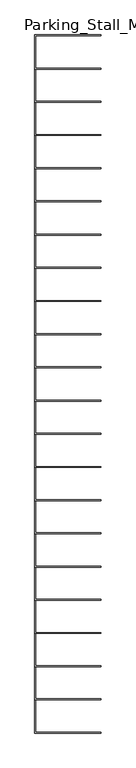
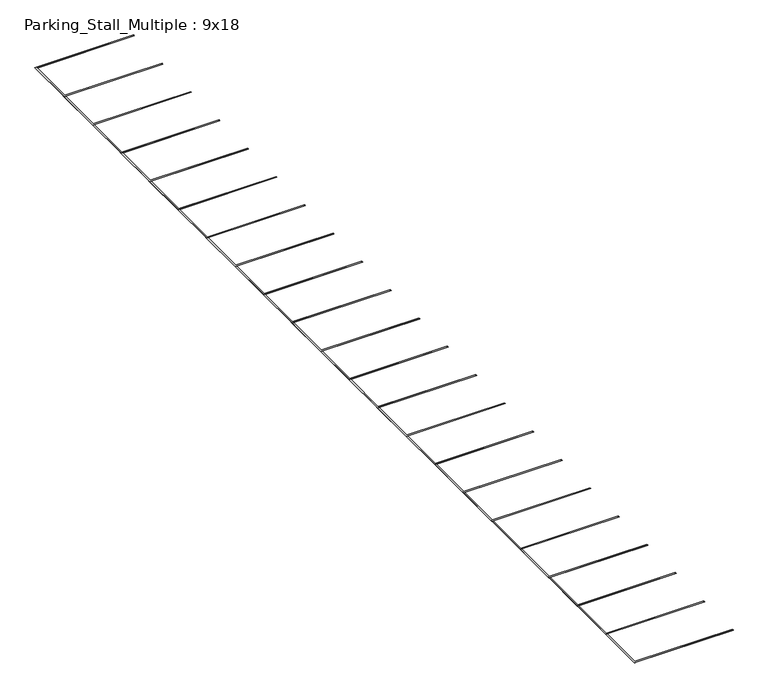
"""IFC4 building model written with IfcOpenShell, lengths in millimetres: proxy geometry, Parking_Stall_Multiple : 9x18."""

from ifc_helpers import new_model, si_unit, origin, origin_with_axes, place, context, project, spatial, polyline, outline, extrude, source, transform, mapped, element, save


def parking_stall_multiple_9x18_b0386777(model_context):
    return source(origin(), model_context, "Body", "SweptSolid", [
        extrude(outline(polyline([(5486.4, 54864.0), (0.0, 54864.0), (0.0, 57683.4), (5486.4, 57683.4), (5486.4, 57607.2), (76.2, 57607.2), (76.2, 54940.2), (5486.4, 54940.2), (5486.4, 54864.0)])), origin_with_axes(), (0.0, 0.0, 1.0), 6.35),
        extrude(outline(polyline([(5486.4, 52120.8), (0.0, 52120.8), (0.0, 54940.2), (5486.4, 54940.2), (5486.4, 54864.0), (76.2, 54864.0), (76.2, 52197.0), (5486.4, 52197.0), (5486.4, 52120.8)])), origin_with_axes(), (0.0, 0.0, 1.0), 6.35),
        extrude(outline(polyline([(5486.4, 49377.6), (0.0, 49377.6), (0.0, 52197.0), (5486.4, 52197.0), (5486.4, 52120.8), (76.2, 52120.8), (76.2, 49453.8), (5486.4, 49453.8), (5486.4, 49377.6)])), origin_with_axes(), (0.0, 0.0, 1.0), 6.35),
        extrude(outline(polyline([(5486.4, 46634.4), (0.0, 46634.4), (0.0, 49453.8), (5486.4, 49453.8), (5486.4, 49377.6), (76.2, 49377.6), (76.2, 46710.6), (5486.4, 46710.6), (5486.4, 46634.4)])), origin_with_axes(), (0.0, 0.0, 1.0), 6.35),
        extrude(outline(polyline([(5486.4, 43891.2), (0.0, 43891.2), (0.0, 46710.6), (5486.4, 46710.6), (5486.4, 46634.4), (76.2, 46634.4), (76.2, 43967.4), (5486.4, 43967.4), (5486.4, 43891.2)])), origin_with_axes(), (0.0, 0.0, 1.0), 6.35),
        extrude(outline(polyline([(5486.4, 41148.0), (0.0, 41148.0), (0.0, 43967.4), (5486.4, 43967.4), (5486.4, 43891.2), (76.2, 43891.2), (76.2, 41224.2), (5486.4, 41224.2), (5486.4, 41148.0)])), origin_with_axes(), (0.0, 0.0, 1.0), 6.35),
        extrude(outline(polyline([(5486.4, 38404.8), (0.0, 38404.8), (0.0, 41224.2), (5486.4, 41224.2), (5486.4, 41148.0), (76.2, 41148.0), (76.2, 38481.0), (5486.4, 38481.0), (5486.4, 38404.8)])), origin_with_axes(), (0.0, 0.0, 1.0), 6.35),
        extrude(outline(polyline([(5486.4, 35661.6), (0.0, 35661.6), (0.0, 38481.0), (5486.4, 38481.0), (5486.4, 38404.8), (76.2, 38404.8), (76.2, 35737.8), (5486.4, 35737.8), (5486.4, 35661.6)])), origin_with_axes(), (0.0, 0.0, 1.0), 6.35),
        extrude(outline(polyline([(5486.4, 32918.4), (0.0, 32918.4), (0.0, 35737.8), (5486.4, 35737.8), (5486.4, 35661.6), (76.2, 35661.6), (76.2, 32994.6), (5486.4, 32994.6), (5486.4, 32918.4)])), origin_with_axes(), (0.0, 0.0, 1.0), 6.35),
        extrude(outline(polyline([(5486.4, 30175.2), (0.0, 30175.2), (0.0, 32994.6), (5486.4, 32994.6), (5486.4, 32918.4), (76.2, 32918.4), (76.2, 30251.4), (5486.4, 30251.4), (5486.4, 30175.2)])), origin_with_axes(), (0.0, 0.0, 1.0), 6.35),
        extrude(outline(polyline([(5486.4, 27432.0), (0.0, 27432.0), (0.0, 30251.4), (5486.4, 30251.4), (5486.4, 30175.2), (76.2, 30175.2), (76.2, 27508.2), (5486.4, 27508.2), (5486.4, 27432.0)])), origin_with_axes(), (0.0, 0.0, 1.0), 6.35),
        extrude(outline(polyline([(5486.4, 24688.8), (0.0, 24688.8), (0.0, 27508.2), (5486.4, 27508.2), (5486.4, 27432.0), (76.2, 27432.0), (76.2, 24765.0), (5486.4, 24765.0), (5486.4, 24688.8)])), origin_with_axes(), (0.0, 0.0, 1.0), 6.35),
        extrude(outline(polyline([(5486.4, 21945.6), (0.0, 21945.6), (0.0, 24765.0), (5486.4, 24765.0), (5486.4, 24688.8), (76.2, 24688.8), (76.2, 22021.8), (5486.4, 22021.8), (5486.4, 21945.6)])), origin_with_axes(), (0.0, 0.0, 1.0), 6.35),
        extrude(outline(polyline([(5486.4, 19202.4), (0.0, 19202.4), (0.0, 22021.8), (5486.4, 22021.8), (5486.4, 21945.6), (76.2, 21945.6), (76.2, 19278.6), (5486.4, 19278.6), (5486.4, 19202.4)])), origin_with_axes(), (0.0, 0.0, 1.0), 6.35),
        extrude(outline(polyline([(5486.4, 16459.2), (0.0, 16459.2), (0.0, 19278.6), (5486.4, 19278.6), (5486.4, 19202.4), (76.2, 19202.4), (76.2, 16535.4), (5486.4, 16535.4), (5486.4, 16459.2)])), origin_with_axes(), (0.0, 0.0, 1.0), 6.35),
        extrude(outline(polyline([(5486.4, 13716.0), (0.0, 13716.0), (0.0, 16535.4), (5486.4, 16535.4), (5486.4, 16459.2), (76.2, 16459.2), (76.2, 13792.2), (5486.4, 13792.2), (5486.4, 13716.0)])), origin_with_axes(), (0.0, 0.0, 1.0), 6.35),
        extrude(outline(polyline([(5486.4, 10972.8), (0.0, 10972.8), (0.0, 13792.2), (5486.4, 13792.2), (5486.4, 13716.0), (76.2, 13716.0), (76.2, 11049.0), (5486.4, 11049.0), (5486.4, 10972.8)])), origin_with_axes(), (0.0, 0.0, 1.0), 6.35),
        extrude(outline(polyline([(5486.4, 8229.6), (0.0, 8229.6), (0.0, 11049.0), (5486.4, 11049.0), (5486.4, 10972.8), (76.2, 10972.8), (76.2, 8305.8), (5486.4, 8305.8), (5486.4, 8229.6)])), origin_with_axes(), (0.0, 0.0, 1.0), 6.35),
        extrude(outline(polyline([(5486.4, 5486.4), (0.0, 5486.4), (0.0, 8305.8), (5486.4, 8305.8), (5486.4, 8229.6), (76.2, 8229.6), (76.2, 5562.6), (5486.4, 5562.6), (5486.4, 5486.4)])), origin_with_axes(), (0.0, 0.0, 1.0), 6.35),
        extrude(outline(polyline([(5486.4, 2743.2), (0.0, 2743.2), (0.0, 5562.6), (5486.4, 5562.6), (5486.4, 5486.4), (76.2, 5486.4), (76.2, 2819.4), (5486.4, 2819.4), (5486.4, 2743.2)])), origin_with_axes(), (0.0, 0.0, 1.0), 6.35),
        extrude(outline(polyline([(5486.4, 0.0), (0.0, 0.0), (0.0, 2819.4), (5486.4, 2819.4), (5486.4, 2743.2), (76.2, 2743.2), (76.2, 76.2), (5486.4, 76.2), (5486.4, 0.0)])), origin_with_axes(), (0.0, 0.0, 1.0), 6.35),
    ])


if __name__ == "__main__":
    model = new_model("IFC4")
    model_context = context("Model", 3, world=origin())
    ifc_project = project(units=[si_unit("LENGTHUNIT", "METRE", prefix="MILLI")], contexts=[model_context])
    site = spatial("IfcSite", under=ifc_project)
    building = spatial("IfcBuilding", under=site)
    placement = place(None, origin())
    parking_stall_multiple_9x18_shape = parking_stall_multiple_9x18_b0386777(model_context)
    element("IfcBuildingElementProxy", 1, Name="Parking_Stall_Multiple : 9x18", ObjectType="Parking_Stall_Multiple : 9x18", at=placement, inside=building, context=model_context, shape_type="MappedRepresentation", body=[
        mapped(parking_stall_multiple_9x18_shape, transform((0.0, 0.0, 0.0), x_axis=(1.0, 0.0, 0.0), y_axis=(0.0, 1.0, 0.0), z_axis=(0.0, 0.0, 1.0))),
    ])
    save(model, "model.ifc")

# Revit data of these elements
# Type "Parking_Stall_Multiple : 9x18"
#   Parking_Width_M = 9' - 0"
#   Parking_Run_Length [instance default] = 65' - 0"
#   Parking_Line_Width = 0' - 3"
#   Parking_Length_M = 18' - 0"
#   Single_Parking_Visibility [instance default] = no
#   Parking_ADA_Symbol = no
#   ParkingUnitsArray [instance default] = 7
#   ParkingUnits [instance default] = 7
#   Multiple_Parking_Visibility [instance default] = yes
#   Parking_Line_Material = none
# Element 1 (IfcBuildingElementProxy, "Parking_Stall_Multiple : 9x18")
#   Parking_Run_Length = 187' - 5.94523"
#   ParkingUnitsArray = 21
#   ParkingUnits = 21
